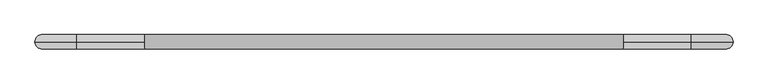
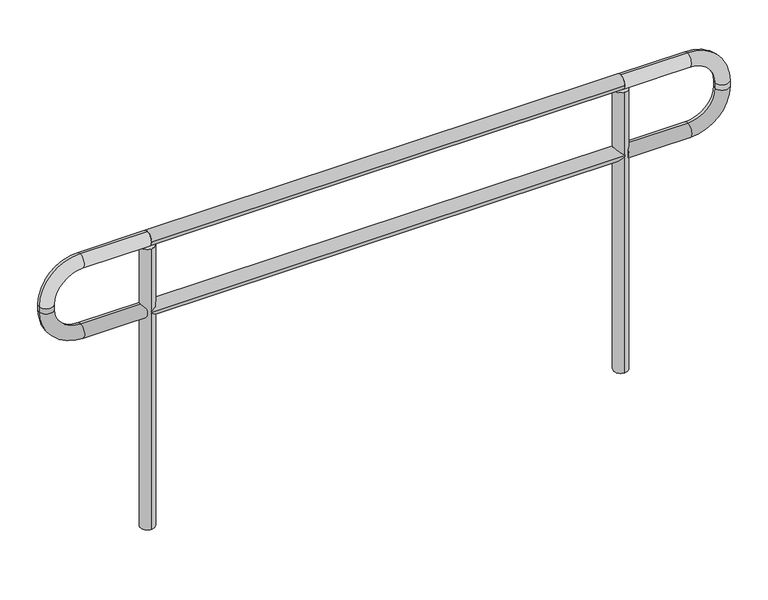
"""IFC4 building model written with IfcOpenShell, lengths in millimetres: railing geometry."""

from ifc_helpers import new_model, si_unit, point, frame, frame_2d, origin, origin_with_axes, place, context, project, spatial, circle_curve, ellipse_curve, trimmed, segment, composite_curve, outline, extrude, source, transform, mapped, element, save
from ifc_brep_helpers import plane_surface, cylinder_surface, revolved_surface, advanced_brep


def railing_16ae2046(model_context):
    return source(origin(), model_context, "Body", "SolidModel", [
        extrude(outline(composite_curve([segment(trimmed(circle_curve(frame_2d((30848.1400611, 899.0)), 21.0), [point((30869.1400611, 899.0))], [point((30827.1400611, 899.0))], False, "CARTESIAN"), True, "CONTINUOUS"), segment(trimmed(circle_curve(frame_2d((30848.1400611, 899.0)), 21.0), [point((30827.1400611, 899.0))], [point((30869.1400611, 899.0))], False, "CARTESIAN"), True, "CONTINUOUS")], self_intersect=False)), frame((9966.6129185, 0.0, 0.0), z_axis=(1.0, 0.0, 0.0), x_axis=(0.0, 1.0, 0.0)), (0.0, 0.0, 1.0), 1400.0),
        extrude(outline(composite_curve([segment(trimmed(circle_curve(frame_2d((30848.1400611, 679.0)), 21.0), [point((30869.1400611, 679.0))], [point((30827.1400611, 679.0))], False, "CARTESIAN"), True, "CONTINUOUS"), segment(trimmed(circle_curve(frame_2d((30848.1400611, 679.0)), 21.0), [point((30827.1400611, 679.0))], [point((30869.1400611, 679.0))], False, "CARTESIAN"), True, "CONTINUOUS")], self_intersect=False)), frame((9966.6129185, 0.0, 0.0), z_axis=(1.0, 0.0, 0.0), x_axis=(0.0, 1.0, 0.0)), (0.0, 0.0, 1.0), 1400.0),
        advanced_brep(
        [(11379.3129185, 30848.1400611, 700.0), (11379.3129185, 30848.1400611, 658.0), (11565.0129185, 30848.1400611, 700.0), (11565.0129185, 30848.1400611, 658.0), (11687.6129185, 30848.1400611, 780.6), (11645.6129185, 30848.1400611, 780.6), (11645.6129185, 30848.1400611, 797.4), (11687.6129185, 30848.1400611, 797.4), (11565.0129185, 30848.1400611, 920.0), (11565.0129185, 30848.1400611, 878.0), (11366.6129185, 30848.1400611, 878.0), (11366.6129185, 30848.1400611, 920.0)],
        [
            (0, 1, circle_curve(frame((11379.3129185, 30848.1400611, 679.0), z_axis=(-1.0, 0.0, 0.0), x_axis=(0.0, 0.0, -1.0)), 21.0)),
            (1, 0, circle_curve(frame((11379.3129185, 30848.1400611, 679.0), z_axis=(-1.0, 0.0, 0.0), x_axis=(0.0, 0.0, -1.0)), 21.0)),
            (0, 2),
            (2, 3, circle_curve(frame((11565.0129185, 30848.1400611, 679.0), z_axis=(-1.0, 0.0, 0.0), x_axis=(0.0, 0.0, -1.0)), 21.0)),
            (3, 1),
            (3, 2, circle_curve(frame((11565.0129185, 30848.1400611, 679.0), z_axis=(-1.0, 0.0, 0.0), x_axis=(0.0, 0.0, -1.0)), 21.0)),
            (4, 3, circle_curve(frame((11565.0129185, 30848.1400611, 780.6), z_axis=(0.0, 1.0, 0.0), x_axis=(0.0, 0.0, -1.0)), 122.6)),
            (2, 5, circle_curve(frame((11565.0129185, 30848.1400611, 780.6), z_axis=(0.0, -1.0, 0.0), x_axis=(0.0, 0.0, -1.0)), 80.6)),
            (5, 4, circle_curve(frame((11666.6129185, 30848.1400611, 780.6), z_axis=(0.0, 0.0, -1.0), x_axis=(1.0, 0.0, 0.0)), 21.0)),
            (4, 5, circle_curve(frame((11666.6129185, 30848.1400611, 780.6), z_axis=(0.0, 0.0, -1.0), x_axis=(1.0, 0.0, 0.0)), 21.0)),
            (5, 6),
            (6, 7, circle_curve(frame((11666.6129185, 30848.1400611, 797.4), z_axis=(0.0, 0.0, -1.0), x_axis=(1.0, 0.0, 0.0)), 21.0)),
            (7, 4),
            (7, 6, circle_curve(frame((11666.6129185, 30848.1400611, 797.4), z_axis=(0.0, 0.0, -1.0), x_axis=(1.0, 0.0, 0.0)), 21.0)),
            (8, 7, circle_curve(frame((11565.0129185, 30848.1400611, 797.4), z_axis=(0.0, 1.0, 0.0), x_axis=(1.0, 0.0, 0.0)), 122.6)),
            (6, 9, circle_curve(frame((11565.0129185, 30848.1400611, 797.4), z_axis=(0.0, -1.0, 0.0), x_axis=(1.0, 0.0, 0.0)), 80.6)),
            (9, 8, circle_curve(frame((11565.0129185, 30848.1400611, 899.0), z_axis=(1.0, 0.0, 0.0), x_axis=(0.0, 0.0, 1.0)), 21.0)),
            (8, 9, circle_curve(frame((11565.0129185, 30848.1400611, 899.0), z_axis=(1.0, 0.0, 0.0), x_axis=(0.0, 0.0, 1.0)), 21.0)),
            (10, 11, circle_curve(frame((11366.6129185, 30848.1400611, 899.0), z_axis=(-1.0, 0.0, 0.0), x_axis=(0.0, 0.0, 1.0)), 21.0)),
            (11, 10, circle_curve(frame((11366.6129185, 30848.1400611, 899.0), z_axis=(-1.0, 0.0, 0.0), x_axis=(0.0, 0.0, 1.0)), 21.0)),
            (9, 10),
            (11, 8),
        ],
        [
            plane_surface(frame((11379.3129185, 30827.1400611, 679.0), z_axis=(-1.0, 0.0, 0.0), x_axis=(0.0, 0.0, -1.0))),
            cylinder_surface(frame((11379.3129185, 30848.1400611, 679.0), z_axis=(-1.0, 0.0, 0.0), x_axis=(0.0, 0.0, -1.0)), 21.0),
            revolved_surface(trimmed(ellipse_curve(frame((11565.0129185, 30848.1400611, 679.0), z_axis=(-1.0, 0.0, 0.0), x_axis=(0.0, 0.0, -1.0)), 21.0, 21.0), [point((11565.0129185, 30848.1400611, 700.0))], [point((11565.0129185, 30848.1400611, 658.0))], True, "CARTESIAN"), (11565.0129185, 30848.1400611, 780.6), (0.0, -1.0, 0.0)),
            revolved_surface(trimmed(ellipse_curve(frame((11565.0129185, 30848.1400611, 679.0), z_axis=(-1.0, 0.0, 0.0), x_axis=(0.0, 0.0, -1.0)), 21.0, 21.0), [point((11565.0129185, 30848.1400611, 658.0))], [point((11565.0129185, 30848.1400611, 700.0))], True, "CARTESIAN"), (11565.0129185, 30848.1400611, 780.6), (0.0, -1.0, 0.0)),
            cylinder_surface(frame((11666.6129185, 30848.1400611, 780.6), z_axis=(0.0, 0.0, -1.0), x_axis=(1.0, 0.0, 0.0)), 21.0),
            revolved_surface(trimmed(ellipse_curve(frame((11666.6129185, 30848.1400611, 797.4), z_axis=(0.0, 0.0, -1.0), x_axis=(1.0, 0.0, 0.0)), 21.0, 21.0), [point((11645.6129185, 30848.1400611, 797.4))], [point((11687.6129185, 30848.1400611, 797.4))], True, "CARTESIAN"), (11565.0129185, 30848.1400611, 797.4), (0.0, -1.0, 0.0)),
            revolved_surface(trimmed(ellipse_curve(frame((11666.6129185, 30848.1400611, 797.4), z_axis=(0.0, 0.0, -1.0), x_axis=(1.0, 0.0, 0.0)), 21.0, 21.0), [point((11687.6129185, 30848.1400611, 797.4))], [point((11645.6129185, 30848.1400611, 797.4))], True, "CARTESIAN"), (11565.0129185, 30848.1400611, 797.4), (0.0, -1.0, 0.0)),
            plane_surface(frame((11366.6129185, 30827.1400611, 899.0), z_axis=(-1.0, 0.0, 0.0), x_axis=(0.0, 0.0, 1.0))),
            cylinder_surface(frame((11565.0129185, 30848.1400611, 899.0), z_axis=(1.0, 0.0, 0.0), x_axis=(0.0, 0.0, 1.0)), 21.0),
        ],
        [
            (0, [[1, 2]]),
            (1, [[-1, 3, 4, 5]]),
            (1, [[-2, -5, 6, -3]]),
            (2, [[7, -4, 8, 9]]),
            (3, [[-8, -6, -7, 10]]),
            (4, [[-9, 11, 12, 13]]),
            (4, [[-10, -13, 14, -11]]),
            (5, [[15, -12, 16, 17]]),
            (6, [[-16, -14, -15, 18]]),
            (7, [[19, 20]]),
            (8, [[-17, 21, -20, 22]]),
            (8, [[-18, -22, -19, -21]]),
        ],
    ),
        extrude(outline(composite_curve([segment(trimmed(circle_curve(frame_2d((11366.6129185, 30848.1400611)), 21.0), [point((11366.6129185, 30827.1400611))], [point((11366.6129185, 30869.1400611))], False, "CARTESIAN"), True, "CONTINUOUS"), segment(trimmed(circle_curve(frame_2d((11366.6129185, 30848.1400611)), 21.0), [point((11366.6129185, 30869.1400611))], [point((11366.6129185, 30827.1400611))], False, "CARTESIAN"), True, "CONTINUOUS")], self_intersect=False)), origin_with_axes(), (0.0, 0.0, 1.0), 878.0),
        advanced_brep(
        [(9966.6129185, 30848.1400611, 878.0), (9966.6129185, 30848.1400611, 920.0), (9768.2129185, 30848.1400611, 878.0), (9768.2129185, 30848.1400611, 920.0), (9645.6129185, 30848.1400611, 797.4), (9687.6129185, 30848.1400611, 797.4), (9687.6129185, 30848.1400611, 780.6), (9645.6129185, 30848.1400611, 780.6), (9768.2129185, 30848.1400611, 658.0), (9768.2129185, 30848.1400611, 700.0), (9953.9129185, 30848.1400611, 700.0), (9953.9129185, 30848.1400611, 658.0)],
        [
            (0, 1, circle_curve(frame((9966.6129185, 30848.1400611, 899.0), z_axis=(1.0, 0.0, 0.0), x_axis=(0.0, 0.0, 1.0)), 21.0)),
            (1, 0, circle_curve(frame((9966.6129185, 30848.1400611, 899.0), z_axis=(1.0, 0.0, 0.0), x_axis=(0.0, 0.0, 1.0)), 21.0)),
            (0, 2),
            (2, 3, circle_curve(frame((9768.2129185, 30848.1400611, 899.0), z_axis=(1.0, 0.0, 0.0), x_axis=(0.0, 0.0, 1.0)), 21.0)),
            (3, 1),
            (3, 2, circle_curve(frame((9768.2129185, 30848.1400611, 899.0), z_axis=(1.0, 0.0, 0.0), x_axis=(0.0, 0.0, 1.0)), 21.0)),
            (4, 3, circle_curve(frame((9768.2129185, 30848.1400611, 797.4), z_axis=(0.0, 1.0, 0.0), x_axis=(0.0, 0.0, 1.0)), 122.6)),
            (2, 5, circle_curve(frame((9768.2129185, 30848.1400611, 797.4), z_axis=(0.0, -1.0, 0.0), x_axis=(0.0, 0.0, 1.0)), 80.6)),
            (5, 4, circle_curve(frame((9666.6129185, 30848.1400611, 797.4), z_axis=(0.0, 0.0, 1.0), x_axis=(-1.0, 0.0, 0.0)), 21.0)),
            (4, 5, circle_curve(frame((9666.6129185, 30848.1400611, 797.4), z_axis=(0.0, 0.0, 1.0), x_axis=(-1.0, 0.0, 0.0)), 21.0)),
            (5, 6),
            (6, 7, circle_curve(frame((9666.6129185, 30848.1400611, 780.6), z_axis=(0.0, 0.0, 1.0), x_axis=(-1.0, 0.0, 0.0)), 21.0)),
            (7, 4),
            (7, 6, circle_curve(frame((9666.6129185, 30848.1400611, 780.6), z_axis=(0.0, 0.0, 1.0), x_axis=(-1.0, 0.0, 0.0)), 21.0)),
            (8, 7, circle_curve(frame((9768.2129185, 30848.1400611, 780.6), z_axis=(0.0, 1.0, 0.0), x_axis=(-1.0, 0.0, 0.0)), 122.6)),
            (6, 9, circle_curve(frame((9768.2129185, 30848.1400611, 780.6), z_axis=(0.0, -1.0, 0.0), x_axis=(-1.0, 0.0, 0.0)), 80.6)),
            (9, 8, circle_curve(frame((9768.2129185, 30848.1400611, 679.0), z_axis=(-1.0, 0.0, 0.0), x_axis=(0.0, 0.0, -1.0)), 21.0)),
            (8, 9, circle_curve(frame((9768.2129185, 30848.1400611, 679.0), z_axis=(-1.0, 0.0, 0.0), x_axis=(0.0, 0.0, -1.0)), 21.0)),
            (10, 11, circle_curve(frame((9953.9129185, 30848.1400611, 679.0), z_axis=(1.0, 0.0, 0.0), x_axis=(0.0, 0.0, -1.0)), 21.0)),
            (11, 10, circle_curve(frame((9953.9129185, 30848.1400611, 679.0), z_axis=(1.0, 0.0, 0.0), x_axis=(0.0, 0.0, -1.0)), 21.0)),
            (9, 10),
            (11, 8),
        ],
        [
            plane_surface(frame((9966.6129185, 30827.1400611, 899.0), z_axis=(1.0, 0.0, 0.0), x_axis=(0.0, 0.0, 1.0))),
            cylinder_surface(frame((9966.6129185, 30848.1400611, 899.0), z_axis=(1.0, 0.0, 0.0), x_axis=(0.0, 0.0, 1.0)), 21.0),
            revolved_surface(trimmed(ellipse_curve(frame((9768.2129185, 30848.1400611, 899.0), z_axis=(1.0, 0.0, 0.0), x_axis=(0.0, 0.0, 1.0)), 21.0, 21.0), [point((9768.2129185, 30848.1400611, 878.0))], [point((9768.2129185, 30848.1400611, 920.0))], True, "CARTESIAN"), (9768.2129185, 30848.1400611, 797.4), (0.0, -1.0, 0.0)),
            revolved_surface(trimmed(ellipse_curve(frame((9768.2129185, 30848.1400611, 899.0), z_axis=(1.0, 0.0, 0.0), x_axis=(0.0, 0.0, 1.0)), 21.0, 21.0), [point((9768.2129185, 30848.1400611, 920.0))], [point((9768.2129185, 30848.1400611, 878.0))], True, "CARTESIAN"), (9768.2129185, 30848.1400611, 797.4), (0.0, -1.0, 0.0)),
            cylinder_surface(frame((9666.6129185, 30848.1400611, 797.4), z_axis=(0.0, 0.0, 1.0), x_axis=(-1.0, 0.0, 0.0)), 21.0),
            revolved_surface(trimmed(ellipse_curve(frame((9666.6129185, 30848.1400611, 780.6), z_axis=(0.0, 0.0, 1.0), x_axis=(-1.0, 0.0, 0.0)), 21.0, 21.0), [point((9687.6129185, 30848.1400611, 780.6))], [point((9645.6129185, 30848.1400611, 780.6))], True, "CARTESIAN"), (9768.2129185, 30848.1400611, 780.6), (0.0, -1.0, 0.0)),
            revolved_surface(trimmed(ellipse_curve(frame((9666.6129185, 30848.1400611, 780.6), z_axis=(0.0, 0.0, 1.0), x_axis=(-1.0, 0.0, 0.0)), 21.0, 21.0), [point((9645.6129185, 30848.1400611, 780.6))], [point((9687.6129185, 30848.1400611, 780.6))], True, "CARTESIAN"), (9768.2129185, 30848.1400611, 780.6), (0.0, -1.0, 0.0)),
            plane_surface(frame((9953.9129185, 30827.1400611, 679.0), z_axis=(1.0, 0.0, 0.0), x_axis=(0.0, 0.0, -1.0))),
            cylinder_surface(frame((9768.2129185, 30848.1400611, 679.0), z_axis=(-1.0, 0.0, 0.0), x_axis=(0.0, 0.0, -1.0)), 21.0),
        ],
        [
            (0, [[1, 2]]),
            (1, [[-1, 3, 4, 5]]),
            (1, [[-2, -5, 6, -3]]),
            (2, [[7, -4, 8, 9]]),
            (3, [[-8, -6, -7, 10]]),
            (4, [[-9, 11, 12, 13]]),
            (4, [[-10, -13, 14, -11]]),
            (5, [[15, -12, 16, 17]]),
            (6, [[-16, -14, -15, 18]]),
            (7, [[19, 20]]),
            (8, [[-17, 21, -20, 22]]),
            (8, [[-18, -22, -19, -21]]),
        ],
    ),
        extrude(outline(composite_curve([segment(trimmed(circle_curve(frame_2d((9966.6129185, 30848.1400611)), 21.0), [point((9966.6129185, 30827.1400611))], [point((9966.6129185, 30869.1400611))], False, "CARTESIAN"), True, "CONTINUOUS"), segment(trimmed(circle_curve(frame_2d((9966.6129185, 30848.1400611)), 21.0), [point((9966.6129185, 30869.1400611))], [point((9966.6129185, 30827.1400611))], False, "CARTESIAN"), True, "CONTINUOUS")], self_intersect=False)), origin_with_axes(), (0.0, 0.0, 1.0), 878.0),
    ])


if __name__ == "__main__":
    model = new_model("IFC4")
    model_context = context("Model", 3, world=origin())
    ifc_project = project(units=[si_unit("LENGTHUNIT", "METRE", prefix="MILLI")], contexts=[model_context])
    site = spatial("IfcSite", under=ifc_project)
    building = spatial("IfcBuilding", under=site)
    placement = place(None, origin())
    railing_shape = railing_16ae2046(model_context)
    element("IfcRailing", 1, at=placement, inside=building, context=model_context, shape_type="MappedRepresentation", body=[
        mapped(railing_shape, transform((0.0, 0.0, 0.0), x_axis=(1.0, 0.0, 0.0), y_axis=(0.0, 1.0, 0.0), z_axis=(0.0, 0.0, 1.0))),
    ])
    save(model, "model.ifc")

# Revit data of these elements
# Element 1 (IfcRailing)
#   Materials on its faces: "Ferro - Pintura Esmalte"
# Materials
#   "Ferro - Pintura Esmalte": class "Pintura", colour RGB 255 255 255, transparency 0, Cost = 0
